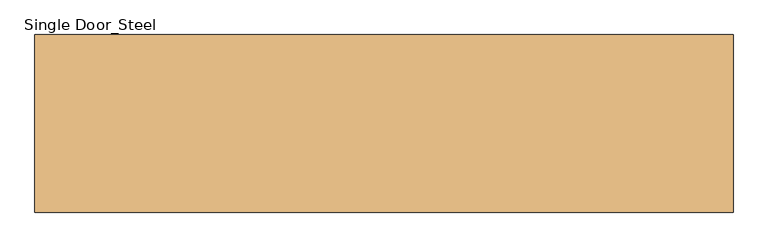
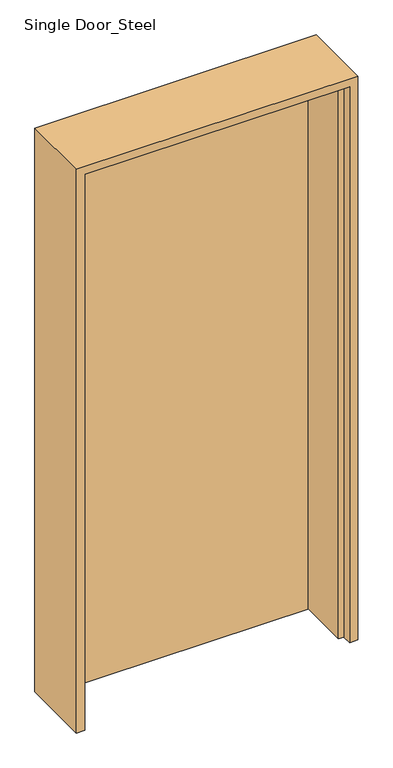
"""IFC4 building model written with IfcOpenShell, lengths in millimetres: door geometry, Single Door_Steel : H_DR_AR B12_Door_Single FSD 01."""

from ifc_helpers import new_model, si_unit, origin, origin_with_axes, place, context, project, spatial, polyline, outline, extrude, faceted_brep, source, transform, mapped, element, save


def single_door_steel_4bf023c6(model_context):
    return source(origin(), model_context, "Body", "SolidModel", [
        extrude(outline(polyline([(480.0, 130.0), (480.0, 95.0), (-480.0, 95.0), (-480.0, 130.0), (480.0, 130.0)])), origin_with_axes(), (0.0, 0.0, 1.0), 2130.0),
        faceted_brep([(480.0, 130.0, 0.0), (510.0, 130.0, 0.0), (510.0, -130.0, 0.0), (480.0, -130.0, 0.0), (480.0, -95.0, 0.0), (460.0, -95.0, 0.0), (460.0, 95.0, 0.0), (480.0, 95.0, 0.0), (480.0, 130.0, 2130.0), (-480.0, 130.0, 2130.0), (-480.0, 130.0, 0.0), (-510.0, 130.0, 0.0), (-510.0, 130.0, 2160.0), (510.0, 130.0, 2160.0), (510.0, -130.0, 2160.0), (-510.0, -130.0, 2160.0), (-510.0, -130.0, 0.0), (-480.0, -130.0, 0.0), (-480.0, -130.0, 2130.0), (480.0, -130.0, 2130.0), (480.0, -95.0, 2130.0), (-480.0, -95.0, 2130.0), (-480.0, -95.0, 0.0), (-460.0, -95.0, 0.0), (-460.0, -95.0, 2110.0), (460.0, -95.0, 2110.0), (460.0, 95.0, 2110.0), (-460.0, 95.0, 2110.0), (-460.0, 95.0, 0.0), (-480.0, 95.0, 0.0), (-480.0, 95.0, 2130.0), (480.0, 95.0, 2130.0)], [[[0, 1, 2, 3, 4, 5, 6, 7]], [[1, 0, 8, 9, 10, 11, 12, 13]], [[2, 1, 13, 14]], [[3, 2, 14, 15, 16, 17, 18, 19]], [[4, 3, 19, 20]], [[5, 4, 20, 21, 22, 23, 24, 25]], [[6, 5, 25, 26]], [[7, 6, 26, 27, 28, 29, 30, 31]], [[0, 7, 31, 8]], [[9, 30, 29, 10]], [[10, 29, 28, 23, 22, 17, 16, 11]], [[15, 12, 11, 16]], [[21, 18, 17, 22]], [[27, 24, 23, 28]], [[14, 13, 12, 15]], [[20, 19, 18, 21]], [[26, 25, 24, 27]], [[8, 31, 30, 9]]]),
    ])


if __name__ == "__main__":
    model = new_model("IFC4")
    model_context = context("Model", 3, world=origin())
    ifc_project = project(units=[si_unit("LENGTHUNIT", "METRE", prefix="MILLI")], contexts=[model_context])
    site = spatial("IfcSite", under=ifc_project)
    building = spatial("IfcBuilding", under=site)
    placement = place(None, origin())
    single_door_steel_shape = single_door_steel_4bf023c6(model_context)
    element("IfcDoor", 1, ObjectType="Single Door_Steel : H_DR_AR B12_Door_Single FSD 01", at=placement, inside=building, context=model_context, shape_type="MappedRepresentation", body=[
        mapped(single_door_steel_shape, transform((0.0, 0.0, 0.0), x_axis=(1.0, 0.0, 0.0), y_axis=(0.0, 1.0, 0.0), z_axis=(0.0, 0.0, 1.0))),
    ])
    save(model, "model.ifc")

# Revit data of these elements
# Type "Single Door_Steel : H_DR_AR B12_Door_Single FSD 01"
#   Type Mark = "FRD"
#   Analytic Construction = "<None>"
#   프레임 투영 외부. = 25 mm
#   프레임 투영 내부. = 25 mm
#   프레임 폭 = 75 mm
#   Height = 2160 mm
#   Width = 1020 mm
#   Define Thermal Properties by = 1
#   문 패널 = none
#   문 프레임 = none
#   Function = (empty or 0)
#   Wall Closure = (empty or 0)
